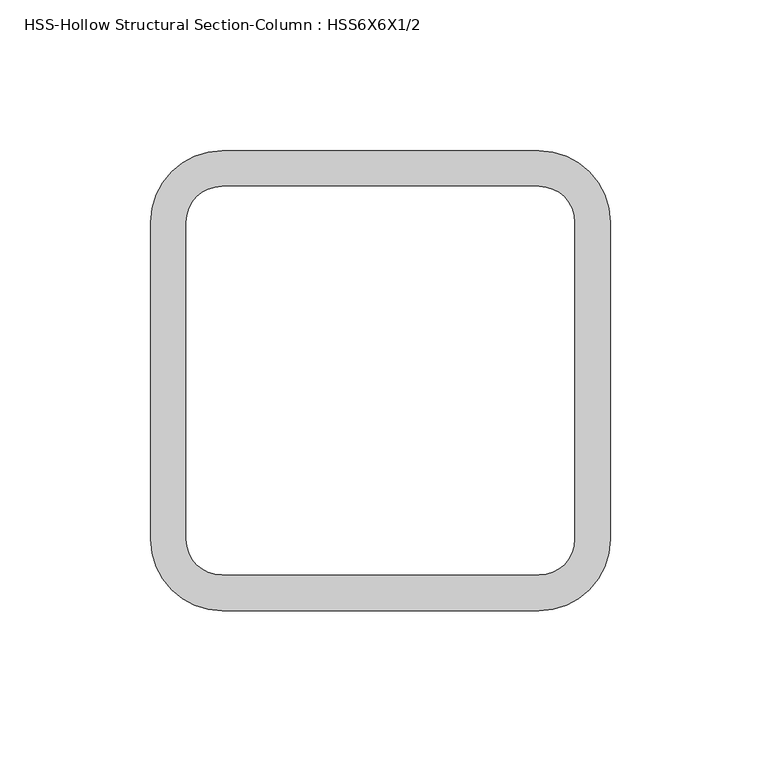
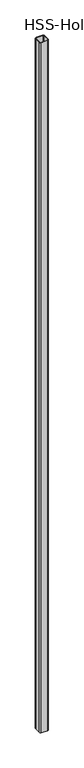
"""IFC4 building model written with IfcOpenShell, lengths in millimetres: column geometry, HSS-Hollow Structural Section-Column : HSS6X6X1/2."""

from ifc_helpers import new_model, si_unit, point, frame_2d, origin, origin_with_axes, place, context, project, spatial, polyline, circle_curve, trimmed, segment, composite_curve, outline, extrude, source, transform, mapped, element, save


def hss_hollow_structural_section_column_hss6x6x1_2_17b669b7(model_context):
    return source(origin(), model_context, "Body", "SweptSolid", [
        extrude(outline(composite_curve([segment(trimmed(circle_curve(frame_2d((52.578, 52.578)), 23.622), [point((52.578, 76.2))], [point((76.2, 52.578))], False, "CARTESIAN"), True, "CONTINUOUS"), segment(polyline([(76.2, 52.578), (76.2, -52.578)]), True, "CONTINUOUS"), segment(trimmed(circle_curve(frame_2d((52.578, -52.578)), 23.622), [point((76.2, -52.578))], [point((52.578, -76.2))], False, "CARTESIAN"), True, "CONTINUOUS"), segment(polyline([(52.578, -76.2), (-52.578, -76.2)]), True, "CONTINUOUS"), segment(trimmed(circle_curve(frame_2d((-52.578, -52.578)), 23.622), [point((-52.578, -76.2))], [point((-76.2, -52.578))], False, "CARTESIAN"), True, "CONTINUOUS"), segment(polyline([(-76.2, -52.578), (-76.2, 52.578)]), True, "CONTINUOUS"), segment(trimmed(circle_curve(frame_2d((-52.578, 52.578)), 23.622), [point((-76.2, 52.578))], [point((-52.578, 76.2))], False, "CARTESIAN"), True, "CONTINUOUS"), segment(polyline([(-52.578, 76.2), (52.578, 76.2)]), True, "CONTINUOUS")], self_intersect=False), holes=[composite_curve([segment(polyline([(52.578, 64.389), (-52.578, 64.389)]), True, "CONTINUOUS"), segment(trimmed(circle_curve(frame_2d((-52.578, 52.578)), 11.811), [point((-52.578, 64.389))], [point((-64.389, 52.578))], True, "CARTESIAN"), True, "CONTINUOUS"), segment(polyline([(-64.389, 52.578), (-64.389, -52.578)]), True, "CONTINUOUS"), segment(trimmed(circle_curve(frame_2d((-52.578, -52.578)), 11.811), [point((-64.389, -52.578))], [point((-52.578, -64.389))], True, "CARTESIAN"), True, "CONTINUOUS"), segment(polyline([(-52.578, -64.389), (52.578, -64.389)]), True, "CONTINUOUS"), segment(trimmed(circle_curve(frame_2d((52.578, -52.578)), 11.811), [point((52.578, -64.389))], [point((64.389, -52.578))], True, "CARTESIAN"), True, "CONTINUOUS"), segment(polyline([(64.389, -52.578), (64.389, 52.578)]), True, "CONTINUOUS"), segment(trimmed(circle_curve(frame_2d((52.578, 52.578)), 11.811), [point((64.389, 52.578))], [point((52.578, 64.389))], True, "CARTESIAN"), True, "CONTINUOUS")], self_intersect=False)]), origin_with_axes(), (0.0, 0.0, 1.0), 12446.0),
    ])


if __name__ == "__main__":
    model = new_model("IFC4")
    model_context = context("Model", 3, world=origin())
    ifc_project = project(units=[si_unit("LENGTHUNIT", "METRE", prefix="MILLI")], contexts=[model_context])
    site = spatial("IfcSite", under=ifc_project)
    building = spatial("IfcBuilding", under=site)
    placement = place(None, origin())
    hss_hollow_structural_section_column_hss6x6x1_2_shape = hss_hollow_structural_section_column_hss6x6x1_2_17b669b7(model_context)
    element("IfcColumn", 1, ObjectType="HSS-Hollow Structural Section-Column : HSS6X6X1/2", at=placement, inside=building, context=model_context, shape_type="MappedRepresentation", body=[
        mapped(hss_hollow_structural_section_column_hss6x6x1_2_shape, transform((0.0, 0.0, 0.0), x_axis=(1.0, 0.0, 0.0), y_axis=(0.0, 1.0, 0.0), z_axis=(0.0, 0.0, 1.0))),
    ])
    save(model, "model.ifc")

# Revit data of these elements
# Type "HSS-Hollow Structural Section-Column : HSS6X6X1/2"
#   Assembly Code = "B10"
#   Shape = "Square"
#   W = 35.1
#   Ht = 0' - 6"
#   b = 0' - 6"
#   kr = 0' - 0.93"
#   t = 0' - 0.465"
#   A = 0.0676389 SF
#   Structural Material [instance default] = Steel ASTM A500, Grade B, Rectangular and Square
# Element 1 (IfcColumn, "HSS-Hollow Structural Section-Column : HSS6X6X1/2")
#   Materials on its faces: "Steel ASTM A500, Grade B, Rectangular and Square"
# Materials
#   "Steel ASTM A500, Grade B, Rectangular and Square": class "Metal", colour RGB 199 199 199, transparency 0, Description = "Carbon steel", Cost = 0
